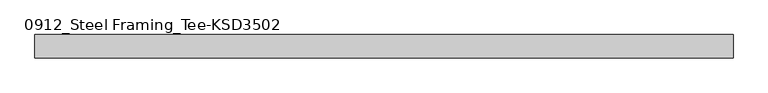
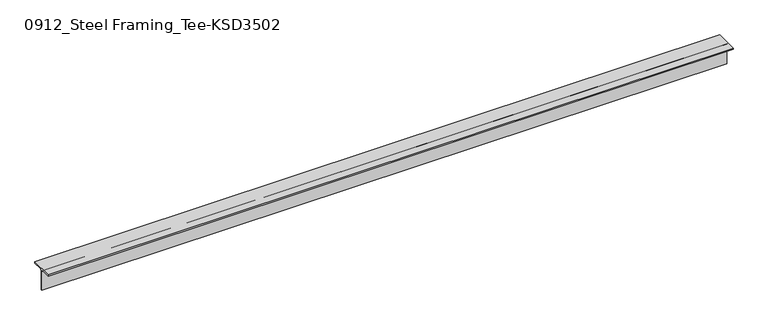
"""IFC4 building model written with IfcOpenShell, lengths in millimetres: member geometry, 0912_Steel Framing_Tee-KSD3502 : H_SB_ASB_CT-150x150x6.5x9."""

from ifc_helpers import new_model, si_unit, point, frame, frame_2d, origin, place, context, project, spatial, polyline, circle_curve, trimmed, segment, composite_curve, outline, extrude, source, transform, mapped, element, save


def member_0912_steel_framing_tee_ksd3502_2a8e7eb1(model_context):
    return source(origin(), model_context, "Body", "SweptSolid", [
        extrude(outline(composite_curve([segment(polyline([(-75.0, 75.0), (75.0, 75.0), (75.0, 66.0), (16.25, 66.0)]), True, "CONTINUOUS"), segment(trimmed(circle_curve(frame_2d((16.25, 53.0)), 13.0), [point((16.25, 66.0))], [point((3.25, 53.0))], True, "CARTESIAN"), True, "CONTINUOUS"), segment(polyline([(3.25, 53.0), (3.25, -75.0), (-3.25, -75.0), (-3.25, 53.0)]), True, "CONTINUOUS"), segment(trimmed(circle_curve(frame_2d((-16.25, 53.0)), 13.0), [point((-3.25, 53.0))], [point((-16.25, 66.0))], True, "CARTESIAN"), True, "CONTINUOUS"), segment(polyline([(-16.25, 66.0), (-75.0, 66.0), (-75.0, 75.0)]), True, "CONTINUOUS")], self_intersect=False)), frame((-2215.2, 0.0, 0.0), z_axis=(1.0, 0.0, 0.0), x_axis=(0.0, 1.0, 0.0)), (0.0, 0.0, 1.0), 4448.4),
    ])


if __name__ == "__main__":
    model = new_model("IFC4")
    model_context = context("Model", 3, world=origin())
    ifc_project = project(units=[si_unit("LENGTHUNIT", "METRE", prefix="MILLI")], contexts=[model_context])
    site = spatial("IfcSite", under=ifc_project)
    building = spatial("IfcBuilding", under=site)
    placement = place(None, origin())
    member_0912_steel_framing_tee_ksd3502_shape = member_0912_steel_framing_tee_ksd3502_2a8e7eb1(model_context)
    element("IfcMember", 1, ObjectType="0912_Steel Framing_Tee-KSD3502 : H_SB_ASB_CT-150x150x6.5x9", at=placement, inside=building, context=model_context, shape_type="MappedRepresentation", body=[
        mapped(member_0912_steel_framing_tee_ksd3502_shape, transform((0.0, 0.0, 0.0), x_axis=(1.0, 0.0, 0.0), y_axis=(0.0, 1.0, 0.0), z_axis=(0.0, 0.0, 1.0))),
    ])
    save(model, "model.ifc")

# Revit data of these elements
# Type "0912_Steel Framing_Tee-KSD3502 : H_SB_ASB_CT-150x150x6.5x9"
#   H_WM Code_1 = "S01AA003-00001 | Main Steel Structure Fabrication Work | Shelter/Building | Light Steel - Standard (30KG/M>Weight) | Material: (   )"
#   H_WM Code_2 = "S03AA029-00001 | Main Steel Structure Erection Work | Shelter/Building | Light Steel (30KG/M>Weight) | Material: (   )"
#   H_WM Code_3 = "S01AA010-00001 | Main Steel Structure Fabrication Work | Shelter/Building | Steel Painting/Coating | for Non-Fireproofed Steel Surface, Surface Preparation, Primer, Second & Final Coat | Material: (   )"
#   H_Q'ty Cal Type Tag = "SB-Q2"
#   Width = 15.0 cm
#   Web Thickness = 0.65 cm
#   Web Fillet = 1.3 cm
#   Section Area = 23.39 cm²
#   Perimeter = 0.60 m²/m
#   Nominal Weight = 18.40 kgf/m
#   Height = 15.0 cm
#   Flange Thickness = 0.9 cm
#   Centroid Vertical = 7.5 cm
#   Centroid Horizontal = 7.5 cm
#   Length [instance default] = 1.5000 m
#   Structural Material [instance default] = Steel, 45-345
#   Warping Constant = (empty or 0)
#   Torsional Moment of Inertia = 0
#   Section Name Key = ""
#   Plastic Modulus weak axis = 0
#   Plastic Modulus strong axis = 0
#   Moment of Inertia weak axis = 0
#   Moment of Inertia strong axis = 0
#   Elastic Modulus weak axis = 0
#   Elastic Modulus strong axis = 0
#   Bolt Spacing = 0
#   Assembly Code = ""
# Element 1 (IfcMember, "0912_Steel Framing_Tee-KSD3502 : H_SB_ASB_CT-150x150x6.5x9")
#   Structural Material = none
# Materials
#   "Steel, 45-345": class "Metal", colour RGB 189 187 185, transparency 0, Description = "Steel 345 MPa", Cost = 0
